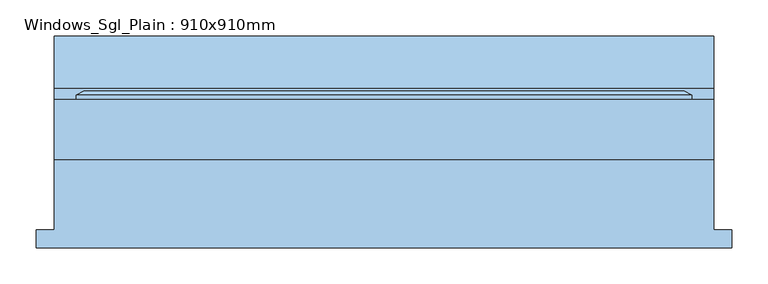
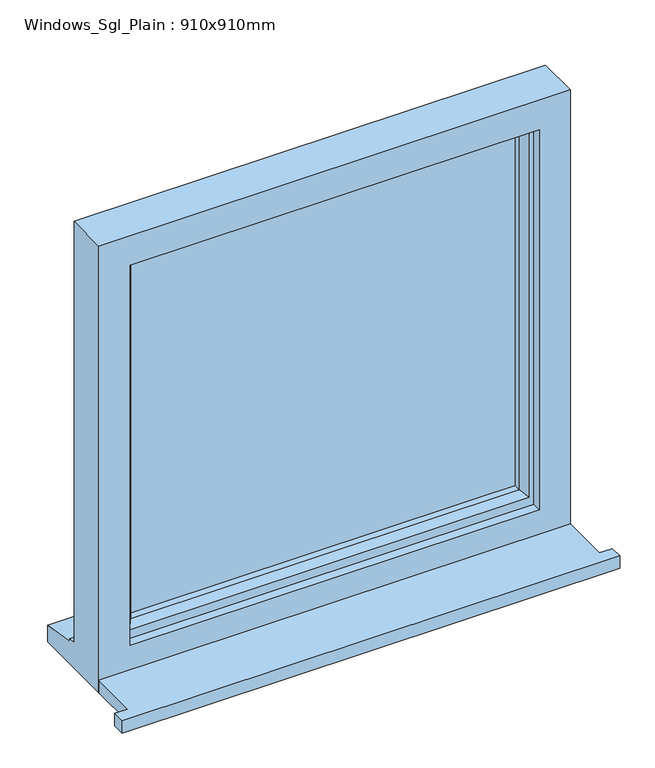
"""IFC4 building model written with IfcOpenShell, lengths in millimetres: window geometry, Windows_Sgl_Plain : 910x910mm."""

from ifc_helpers import new_model, si_unit, frame, origin, place, context, project, spatial, polyline, outline, extrude, faceted_brep, source, transform, mapped, element, save


def windows_sgl_plain_910x910mm_b310e7d5(model_context):
    return source(origin(), model_context, "Body", "SolidModel", [
        extrude(outline(polyline([(-480.0, -131.5434322), (-480.0, -106.5434322), (-455.0, -106.5434322), (-455.0, -9.5434322), (455.0, -9.5434322), (455.0, -106.5434322), (480.0, -106.5434322), (480.0, -131.5434322), (-480.0, -131.5434322)])), frame((0.0, 0.0, 1200.0), z_axis=(0.0, 0.0, 1.0), x_axis=(1.0, 0.0, 0.0)), (0.0, 0.0, 1.0), 25.0),
        faceted_brep([(-455.0, -9.5434322, 1200.0), (455.0, -9.5434322, 1200.0), (455.0, -9.5434322, 2110.0), (-455.0, -9.5434322, 2110.0), (-395.0, -9.5434322, 2050.0), (395.0, -9.5434322, 2050.0), (395.0, -9.5434322, 1275.0), (-395.0, -9.5434322, 1275.0), (-455.0, 73.4565678, 2110.0), (-455.0, 73.4565678, 1251.0), (-455.0, 88.4565678, 1249.68767), (-455.0, 88.4565678, 1244.7449676), (-455.0, 160.9565678, 1233.8088847), (-455.0, 160.9565678, 1200.0), (455.0, 73.4565678, 2110.0), (455.0, 73.4565678, 1251.0), (-415.0, 73.4565678, 2070.0), (-415.0, 73.4565678, 1263.0), (415.0, 73.4565678, 1263.0), (415.0, 73.4565678, 2070.0), (-415.0, 8.4565678, 2070.0), (-415.0, 8.4565678, 1263.0), (415.0, 8.4565678, 2070.0), (415.0, 8.4565678, 1263.0), (-395.0, 8.4565678, 2050.0), (-395.0, 8.4565678, 1275.0), (395.0, 8.4565678, 1275.0), (395.0, 8.4565678, 2050.0), (455.0, 160.9565678, 1200.0), (455.0, 160.9565678, 1233.8088847), (455.0, 88.4565678, 1244.7449676), (455.0, 88.4565678, 1249.68767)], [[[0, 1, 2, 3], [4, 5, 6, 7]], [[0, 3, 8, 9, 10, 11, 12, 13]], [[9, 8, 14, 15], [16, 17, 18, 19]], [[17, 16, 20, 21]], [[20, 22, 23, 21], [24, 25, 26, 27]], [[24, 4, 7, 25]], [[3, 2, 14, 8]], [[16, 19, 22, 20]], [[5, 4, 24, 27]], [[15, 14, 2, 1, 28, 29, 30, 31]], [[19, 18, 23, 22]], [[5, 27, 26, 6]], [[28, 1, 0, 13]], [[29, 28, 13, 12]], [[30, 29, 12, 11]], [[31, 30, 11, 10]], [[15, 31, 10, 9]], [[21, 23, 18, 17]], [[7, 6, 26, 25]]]),
        extrude(outline(polyline([(385.0, 37.4565678), (-385.0, 37.4565678), (-385.0, 61.4565678), (385.0, 61.4565678), (385.0, 37.4565678)])), frame((0.0, 0.0, 1293.0), z_axis=(0.0, 0.0, 1.0), x_axis=(1.0, 0.0, 0.0)), (0.0, 0.0, 1.0), 747.0),
        faceted_brep([(-425.0, 73.4565678, 2080.0), (-425.0, 79.2300705, 2080.0), (-425.0, 79.2300705, 1253.0), (-425.0, 73.4565678, 1253.0), (-415.0, 8.4565678, 2070.0), (-415.0, 73.4565678, 2070.0), (-415.0, 73.4565678, 1263.0), (-415.0, 8.4565678, 1263.0), (-375.0, 22.9494677, 2030.0), (-385.1480377, 8.4565678, 2040.1480377), (-385.1480377, 8.4565678, 1292.8519623), (-375.0, 22.9494677, 1303.0), (-375.0, 37.4565678, 2030.0), (-375.0, 37.4565678, 1303.0), (-385.0, 61.4565678, 2040.0), (-385.0, 37.4565678, 2040.0), (-385.0, 37.4565678, 1293.0), (-385.0, 61.4565678, 1293.0), (-375.0, 79.2300705, 2030.0), (-375.0, 61.4565678, 2030.0), (-375.0, 61.4565678, 1303.0), (-375.0, 79.2300705, 1303.0), (-392.4457548, 85.0035732, 2047.4457548), (-392.4457548, 85.0035732, 1285.5542452), (-414.2153903, 85.0035732, 2069.2153903), (-414.2153903, 85.0035732, 1263.7846097), (425.0, 79.2300705, 1253.0), (425.0, 73.4565678, 1253.0), (415.0, 73.4565678, 1263.0), (415.0, 8.4565678, 1263.0), (385.1480377, 8.4565678, 1292.8519623), (375.0, 22.9494677, 1303.0), (375.0, 37.4565678, 1303.0), (385.0, 37.4565678, 1293.0), (385.0, 61.4565678, 1293.0), (375.0, 61.4565678, 1303.0), (375.0, 79.2300705, 1303.0), (392.4457548, 85.0035732, 1285.5542452), (414.2153903, 85.0035732, 1263.7846097), (425.0, 79.2300705, 2080.0), (425.0, 73.4565678, 2080.0), (415.0, 73.4565678, 2070.0), (415.0, 8.4565678, 2070.0), (385.1480377, 8.4565678, 2040.1480377), (375.0, 22.9494677, 2030.0), (375.0, 37.4565678, 2030.0), (385.0, 37.4565678, 2040.0), (385.0, 61.4565678, 2040.0), (375.0, 61.4565678, 2030.0), (375.0, 79.2300705, 2030.0), (392.4457548, 85.0035732, 2047.4457548), (414.2153903, 85.0035732, 2069.2153903)], [[[0, 1, 2, 3]], [[4, 5, 6, 7]], [[8, 9, 10, 11]], [[12, 8, 11, 13]], [[14, 15, 16, 17]], [[18, 19, 20, 21]], [[22, 18, 21, 23]], [[1, 24, 25, 2]], [[3, 2, 26, 27]], [[7, 6, 28, 29]], [[11, 10, 30, 31]], [[13, 11, 31, 32]], [[17, 16, 33, 34]], [[21, 20, 35, 36]], [[23, 21, 36, 37]], [[2, 25, 38, 26]], [[27, 26, 39, 40]], [[29, 28, 41, 42]], [[31, 30, 43, 44]], [[32, 31, 44, 45]], [[34, 33, 46, 47]], [[36, 35, 48, 49]], [[37, 36, 49, 50]], [[26, 38, 51, 39]], [[40, 39, 1, 0]], [[3, 27, 40, 0], [5, 41, 28, 6]], [[42, 41, 5, 4]], [[7, 29, 42, 4], [9, 43, 30, 10]], [[44, 43, 9, 8]], [[45, 44, 8, 12]], [[15, 46, 33, 16], [13, 32, 45, 12]], [[47, 46, 15, 14]], [[17, 34, 47, 14], [19, 48, 35, 20]], [[49, 48, 19, 18]], [[50, 49, 18, 22]], [[24, 51, 38, 25], [23, 37, 50, 22]], [[39, 51, 24, 1]]]),
    ])


if __name__ == "__main__":
    model = new_model("IFC4")
    model_context = context("Model", 3, world=origin())
    ifc_project = project(units=[si_unit("LENGTHUNIT", "METRE", prefix="MILLI")], contexts=[model_context])
    site = spatial("IfcSite", under=ifc_project)
    building = spatial("IfcBuilding", under=site)
    placement = place(None, origin())
    windows_sgl_plain_910x910mm_shape = windows_sgl_plain_910x910mm_b310e7d5(model_context)
    element("IfcWindow", 1, ObjectType="Windows_Sgl_Plain : 910x910mm", at=placement, inside=building, context=model_context, shape_type="MappedRepresentation", body=[
        mapped(windows_sgl_plain_910x910mm_shape, transform((0.0, 0.0, 0.0), x_axis=(1.0, 0.0, 0.0), y_axis=(0.0, 1.0, 0.0), z_axis=(0.0, 0.0, 1.0))),
    ])
    save(model, "model.ifc")

# Revit data of these elements
# Type "Windows_Sgl_Plain : 910x910mm"
#   Type Mark = "44"
#   Operation = "SinglePanel"
#   Construction Type Id = "SGL"
#   Manufacturer = "Revit"
#   Keynote = "L10"
#   Analytic Construction = "Large single-glazed windows"
#   Wrap Layers (Ext) from Ext = 102.5 mm
#   Wrap Layers (Int) from Ext = 177.5 mm
#   Window Board Projection = 25 mm
#   Window Board Extension = 25 mm
#   Visual Light Transmittance = 0.9
#   Solar Heat Gain Coefficient = 0.86
#   Rough Width = 910 mm
#   Rough Height = 910 mm
#   Height = 910 mm
#   Width = 910 mm
#   Heat Transfer Coefficient (U) = 5.5617 W/(m²·K)
#   Glazing Thickness = 24 mm
#   FrameOffset - External = 50 mm
#   Frame Depth = 65 mm
#   Default Head Height = 2110 mm
#   Cill Depth = 87.5 mm
#   Cavity Closer Width = 50 mm
#   Cavity Closer Offset from Ext = 102.5 mm
#   Cavity Closer Depth = 85 mm
#   Define Thermal Properties by = 1
#   Vis - Cavity Closers = yes
#   Define Thermal Properties by = 1
#   Material Trim = Window Frame
#   Material Glass = Glass
#   Material Frame = Window Frame
#   Wall Closure = (empty or 0)
# Element 1 (IfcWindow, "Windows_Sgl_Plain : 910x910mm")
#   Materials on its faces: "Window Frame", "Glass"
# Materials
#   "Window Frame": class "Miscellaneous", colour RGB 249 249 249, transparency 0, Keynote = "L10", Cost = 0
#   "Glass": class "Glass", colour RGB 0 128 192, transparency 0.9, Description = "Soda Lime Glass", Cost = 0
